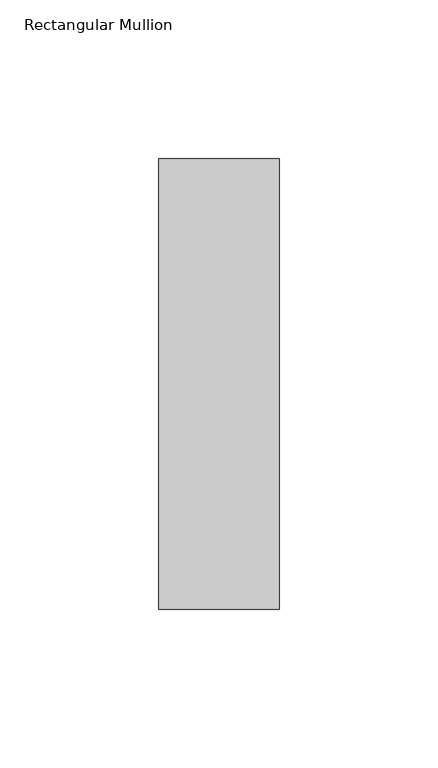
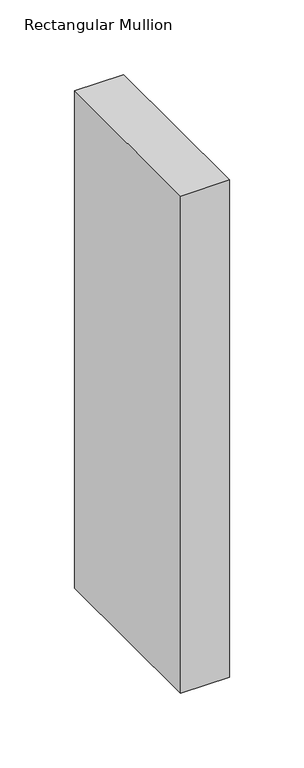
"""IFC4 building model written with IfcOpenShell, lengths in millimetres: member geometry, Rectangular Mullion : NLRS_21_CWM_hsb-regel 38x142_gen_rsf."""

from ifc_helpers import new_model, si_unit, frame, origin, place, context, project, spatial, polyline, outline, extrude, source, transform, mapped, element, save


def rectangular_mullion_b195b317(model_context):
    return source(origin(), model_context, "Body", "SweptSolid", [
        extrude(outline(polyline([(-38.0, -71.0), (-38.0, 71.0), (0.0, 71.0), (0.0, -71.0), (-38.0, -71.0)])), frame((0.0, 0.0, -407.0000003), z_axis=(0.0, 0.0, 1.0), x_axis=(1.0, 0.0, 0.0)), (0.0, 0.0, 1.0), 407.0000003),
    ])


if __name__ == "__main__":
    model = new_model("IFC4")
    model_context = context("Model", 3, world=origin())
    ifc_project = project(units=[si_unit("LENGTHUNIT", "METRE", prefix="MILLI")], contexts=[model_context])
    site = spatial("IfcSite", under=ifc_project)
    building = spatial("IfcBuilding", under=site)
    placement = place(None, origin())
    rectangular_mullion_shape = rectangular_mullion_b195b317(model_context)
    element("IfcMember", 1, ObjectType="Rectangular Mullion : NLRS_21_CWM_hsb-regel 38x142_gen_rsf", at=placement, inside=building, context=model_context, shape_type="MappedRepresentation", body=[
        mapped(rectangular_mullion_shape, transform((0.0, 0.0, 0.0), x_axis=(1.0, 0.0, 0.0), y_axis=(0.0, 1.0, 0.0), z_axis=(0.0, 0.0, 1.0))),
    ])
    save(model, "model.ifc")

# Revit data of these elements
# Type "Rectangular Mullion : NLRS_21_CWM_hsb-regel 38x142_gen_rsf"
#   Export Type to IFC As = "IfcWall"
#   Type IfcGUID = "07M7mRoiH1CR8m_RSKIwpF"
#   Assembly Code = "21.10"
#   built-in parameter 1007322 = 0.465879 (stored number, unit not read)
#   built-in parameter 1007321 = 0.062336 (stored number, unit not read)
#   built-in parameter 1007320 = 0.062336 (stored number, unit not read)
# Element 1 (IfcMember, "Rectangular Mullion : NLRS_21_CWM_hsb-regel 38x142_gen_rsf")
#   Materials on its faces: "NLRS_i2_hout naaldhout vuren_gen_rsf"
# Materials
#   "NLRS_i2_hout naaldhout vuren_gen_rsf": class "I - Hout", colour RGB 234 199 147, transparency 0, Keynote = "i2", Manufacturer = "Revit Standards Foundation", URL = "www.revitstandards.org", Description = "hout vuren", Cost = 0
